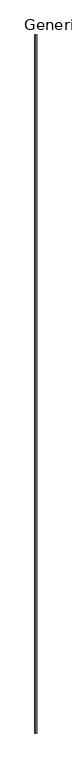
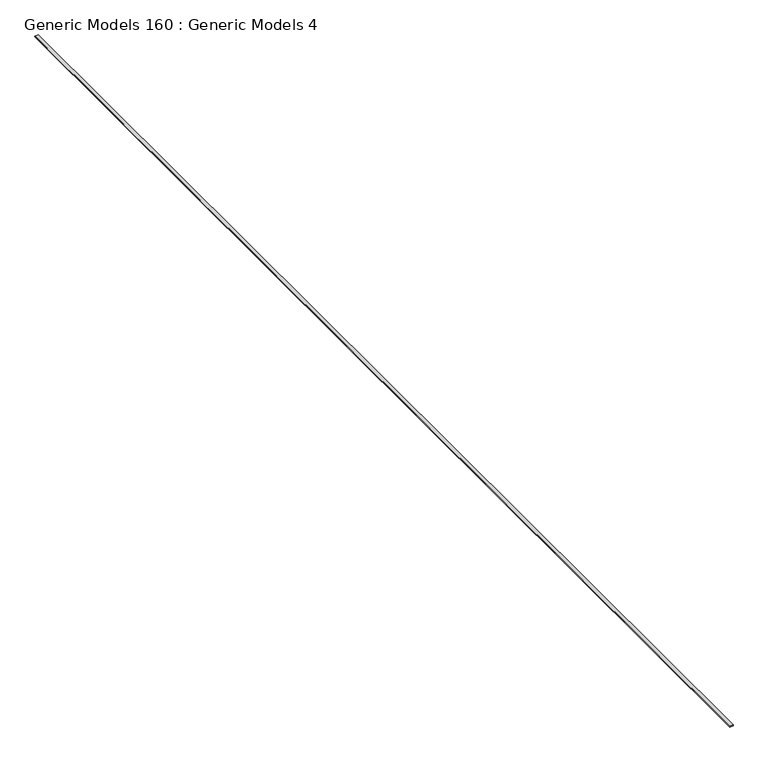
"""IFC4 building model written with IfcOpenShell, lengths in millimetres: proxy geometry, Generic Models 160 : Generic Models 4."""

import ifcopenshell
import ifcopenshell.guid

model = None  # the IFC model being written
_history = None  # IfcOwnerHistory: only IFC2X3 demands one
_inside = {}  # id of a spatial element -> (the spatial element, [elements in it])
_under = {}  # id of a project, library or spatial element -> (it, [spatial elements below it])
_declared = {}  # id of a project -> (the project, [libraries it declares])
_typed = {}  # id of a type object -> (the type object, [elements of that type])
_made_of = {}  # id of a material, layer set ... -> (it, [elements and type objects made of it])


def new_model(schema):
    """Start an empty IFC model of exactly this schema.

    Asked for "IFC4X3", IfcOpenShell would pick the latest addendum, in which some entities
    have other attributes; the version numbers below select the first issue.
    IFC2X3 requires an IfcOwnerHistory on every rooted entity: one is made here for all.
    """
    global model, _history
    if schema == "IFC4X3":
        model = ifcopenshell.file(schema_version=(4, 3, 0, 0))
    else:
        model = ifcopenshell.file(schema=schema)
    _inside.clear()
    _under.clear()
    _declared.clear()
    _typed.clear()
    _made_of.clear()
    _history = None
    if model.schema == "IFC2X3":
        org = make("IfcOrganization", Name="unknown")
        user = make(
            "IfcPersonAndOrganization",
            ThePerson=make("IfcPerson", FamilyName="unknown"),
            TheOrganization=org,
        )
        app = make(
            "IfcApplication",
            ApplicationDeveloper=org,
            Version="unknown",
            ApplicationFullName="unknown",
            ApplicationIdentifier="unknown",
        )
        _history = make(
            "IfcOwnerHistory",
            OwningUser=user,
            OwningApplication=app,
            ChangeAction="ADDED",
            CreationDate=0,
        )
    return model


def make(cls, **values):
    """One entity of the class cls with the attributes given. An attribute that is None is left unset."""
    return model.create_entity(
        cls, **{name: value for name, value in values.items() if value is not None}
    )


def rooted(cls, **values):
    """An entity with a GlobalId (a new one), such as an element, a storey or a relation."""
    return make(cls, GlobalId=ifcopenshell.guid.new(), OwnerHistory=_history, **values)


def si_unit(unit_type, name, prefix=None):
    """IfcSIUnit, for example si_unit("LENGTHUNIT", "METRE", prefix="MILLI")."""
    return make("IfcSIUnit", UnitType=unit_type, Prefix=prefix, Name=name)


def assignment(units):
    """IfcUnitAssignment: the units of a project."""
    return None if units is None else make("IfcUnitAssignment", Units=units)


def point(xyz):
    """IfcCartesianPoint."""
    return None if xyz is None else make("IfcCartesianPoint", Coordinates=xyz)


def direction(xyz):
    """IfcDirection."""
    return None if xyz is None else make("IfcDirection", DirectionRatios=xyz)


def frame(location, z_axis=None, x_axis=None):
    """IfcAxis2Placement3D, a coordinate frame: its origin and axes. An axis left out is left unset."""
    return make(
        "IfcAxis2Placement3D",
        Location=point(location),
        Axis=direction(z_axis),
        RefDirection=direction(x_axis),
    )


def frame_2d(location, x_axis=None):
    """IfcAxis2Placement2D, a coordinate frame in the plane: its origin and x axis."""
    return make(
        "IfcAxis2Placement2D", Location=point(location), RefDirection=direction(x_axis)
    )


def origin():
    """The frame at (0, 0, 0) with its axes left unset."""
    return frame((0.0, 0.0, 0.0))


def place(relative_to, where):
    """IfcLocalPlacement: puts the frame where relative to a parent placement (None: the world)."""
    return make(
        "IfcLocalPlacement", PlacementRelTo=relative_to, RelativePlacement=where
    )


def context(
    kind, dimensions, precision=None, world=None, true_north=None, identifier=None
):
    """IfcGeometricRepresentationContext, for example the 3D "Model" context."""
    return make(
        "IfcGeometricRepresentationContext",
        ContextIdentifier=identifier,
        ContextType=kind,
        CoordinateSpaceDimension=dimensions,
        Precision=precision,
        WorldCoordinateSystem=world,
        TrueNorth=true_north,
    )


def project(units=None, contexts=None):
    """IfcProject with its units and contexts."""
    return rooted(
        "IfcProject",
        Name="project",
        RepresentationContexts=contexts,
        UnitsInContext=assignment(units),
    )


def spatial(cls, under=None, at=None, **own):
    """A site, building, storey or space (cls), placed at a placement, below another one or the project."""
    s = rooted(cls, ObjectPlacement=at, **own)
    if under is not None:
        _under.setdefault(under.id(), (under, []))[1].append(s)
    return s


def polyline(points):
    """IfcPolyline through the points."""
    return make("IfcPolyline", Points=[point(p) for p in points])


def circle_curve(where, radius):
    """IfcCircle in the frame where."""
    return make("IfcCircle", Position=where, Radius=radius)


def trimmed(basis, trim1, trim2, sense, master):
    """IfcTrimmedCurve: the piece of a basis curve between two trims."""
    return make(
        "IfcTrimmedCurve",
        BasisCurve=basis,
        Trim1=trim1,
        Trim2=trim2,
        SenseAgreement=sense,
        MasterRepresentation=master,
    )


def segment(curve, same_sense, transition):
    """IfcCompositeCurveSegment."""
    return make(
        "IfcCompositeCurveSegment",
        Transition=transition,
        SameSense=same_sense,
        ParentCurve=curve,
    )


def composite_curve(segments, self_intersect=None):
    """IfcCompositeCurve: segments joined end to end."""
    return make("IfcCompositeCurve", Segments=segments, SelfIntersect=self_intersect)


def outline(outer, holes=None, kind="AREA"):
    """IfcArbitraryClosedProfileDef: a profile drawn as a closed curve; with holes, ...WithVoids."""
    if holes is None:
        return make("IfcArbitraryClosedProfileDef", ProfileType=kind, OuterCurve=outer)
    return make(
        "IfcArbitraryProfileDefWithVoids",
        ProfileType=kind,
        OuterCurve=outer,
        InnerCurves=holes,
    )


def extrude(swept, where, along, depth):
    """IfcExtrudedAreaSolid: the profile swept, set in the frame where, extruded along a direction by depth."""
    return make(
        "IfcExtrudedAreaSolid",
        SweptArea=swept,
        Position=where,
        ExtrudedDirection=direction(along),
        Depth=depth,
    )


def shape(context_of_items, identifier, shape_type, items):
    """IfcShapeRepresentation: the items that make up one representation, for example the "Body"."""
    return make(
        "IfcShapeRepresentation",
        ContextOfItems=context_of_items,
        RepresentationIdentifier=identifier,
        RepresentationType=shape_type,
        Items=items,
    )


def source(mapping_origin, context_of_items, identifier, shape_type, items):
    """IfcRepresentationMap: a shape defined once, which mapped items show again and again."""
    return make(
        "IfcRepresentationMap",
        MappingOrigin=mapping_origin,
        MappedRepresentation=shape(context_of_items, identifier, shape_type, items),
    )


def transform(
    local_origin,
    x_axis=None,
    y_axis=None,
    z_axis=None,
    scale=None,
    scale2=None,
    scale3=None,
    uniform=True,
):
    """IfcCartesianTransformationOperator3D, or its non-uniform kind. x_axis, y_axis, z_axis: its Axis1, 2, 3."""
    if uniform:
        return make(
            "IfcCartesianTransformationOperator3D",
            Axis1=direction(x_axis),
            Axis2=direction(y_axis),
            LocalOrigin=point(local_origin),
            Scale=scale,
            Axis3=direction(z_axis),
        )
    return make(
        "IfcCartesianTransformationOperator3DnonUniform",
        Axis1=direction(x_axis),
        Axis2=direction(y_axis),
        LocalOrigin=point(local_origin),
        Scale=scale,
        Axis3=direction(z_axis),
        Scale2=scale2,
        Scale3=scale3,
    )


def mapped(mapping_source, mapping_target):
    """IfcMappedItem: shows the shape of a source again, moved by a transform."""
    return make(
        "IfcMappedItem", MappingSource=mapping_source, MappingTarget=mapping_target
    )


def made_of(thing, what):
    """Note that an element or type object is made of a material, layer set ...; save() writes the relation."""
    if what is not None:
        _made_of.setdefault(what.id(), (what, []))[1].append(thing)
    return thing


def element(
    cls,
    number,
    at=None,
    inside=None,
    cuts=None,
    type_object=None,
    material=None,
    context=None,
    identifier="Body",
    shape_type=None,
    held_by="IfcProductDefinitionShape",
    body=None,
    shapes=None,
    **own,
):
    """One element of the class cls, such as IfcWall. Its Tag is "e" and its number.

    at: its placement. inside: the storey or other place that contains it. cuts: it is an
    opening in that element (IfcRelVoidsElement). A single representation is given by context,
    identifier, shape_type and body (its items); several are given by shapes. held_by: the class
    of the entity that holds the representations. save() writes the other relations.
    """
    e = rooted(cls, Tag="e%d" % number, ObjectPlacement=at, **own)
    if body is not None:
        shapes = [shape(context, identifier, shape_type, body)]
    if shapes is not None:
        e.Representation = make(held_by, Representations=shapes)
    if inside is not None:
        _inside.setdefault(inside.id(), (inside, []))[1].append(e)
    if cuts is not None:
        rooted(
            "IfcRelVoidsElement", RelatingBuildingElement=cuts, RelatedOpeningElement=e
        )
    if type_object is not None:
        _typed.setdefault(type_object.id(), (type_object, []))[1].append(e)
    return made_of(e, material)


def aggregate(whole, parts):
    """IfcRelAggregates: a whole, such as a stair, and the parts it consists of."""
    return rooted("IfcRelAggregates", RelatingObject=whole, RelatedObjects=parts)


def save(model, path):
    """Write the relations noted so far, then the file.

    IfcRelAggregates (storeys below a building ...), IfcRelContainedInSpatialStructure (elements
    in a storey), IfcRelDefinesByType, IfcRelAssociatesMaterial and IfcRelDeclares: one each for
    every whole, place, type object, material and project.
    """
    for whole, parts in _under.values():
        aggregate(whole, parts)
    for where, things in _inside.values():
        rooted(
            "IfcRelContainedInSpatialStructure",
            RelatedElements=things,
            RelatingStructure=where,
        )
    for kind, things in _typed.values():
        rooted("IfcRelDefinesByType", RelatedObjects=things, RelatingType=kind)
    for what, things in _made_of.values():
        rooted("IfcRelAssociatesMaterial", RelatedObjects=things, RelatingMaterial=what)
    for by, libraries in _declared.values():
        rooted("IfcRelDeclares", RelatingContext=by, RelatedDefinitions=libraries)
    model.write(path)


def generic_models_160_generic_models_4_b938c61c(model_context):
    return source(origin(), model_context, "Body", "SweptSolid", [
        extrude(outline(composite_curve([segment(trimmed(circle_curve(frame_2d((122788.9609874, -10292.4988366)), 5.3394144), [point((122793.7234874, -10290.0847239))], [point((122784.1984874, -10290.0847239))], True, "CARTESIAN"), True, "CONTINUOUS"), segment(polyline([(122784.1984874, -10290.0847239), (122784.1984874, -10252.9339552), (122793.7234874, -10252.9339552), (122793.7234874, -10290.0847239)]), True, "CONTINUOUS")], self_intersect=False)), frame((0.0, -5493.3230338, 0.0), z_axis=(0.0, 1.0, 0.0), x_axis=(0.0, 0.0, 1.0)), (0.0, 0.0, 1.0), 12547.6),
    ])


if __name__ == "__main__":
    model = new_model("IFC4")
    model_context = context("Model", 3, world=origin())
    ifc_project = project(units=[si_unit("LENGTHUNIT", "METRE", prefix="MILLI")], contexts=[model_context])
    site = spatial("IfcSite", under=ifc_project)
    building = spatial("IfcBuilding", under=site)
    placement = place(None, origin())
    generic_models_160_generic_models_4_shape = generic_models_160_generic_models_4_b938c61c(model_context)
    element("IfcBuildingElementProxy", 1, Name="Generic Models 160 : Generic Models 4", ObjectType="Generic Models 160 : Generic Models 4", at=placement, inside=building, context=model_context, shape_type="MappedRepresentation", body=[
        mapped(generic_models_160_generic_models_4_shape, transform((0.0, 0.0, 0.0), x_axis=(1.0, 0.0, 0.0), y_axis=(0.0, 1.0, 0.0), z_axis=(0.0, 0.0, 1.0))),
    ])
    save(model, "model.ifc")

# Revit data of these elements
# Element 1 (IfcBuildingElementProxy, "Generic Models 160 : Generic Models 4")
#   Materials on its faces: "_MORTAR SETTING BED"
# Materials
#   "_MORTAR SETTING BED": class "Generic", colour RGB 191 191 191, transparency 0, Cost = 0
